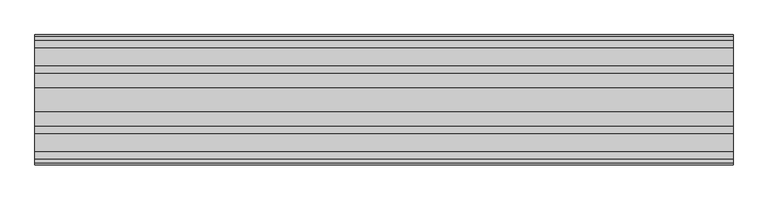
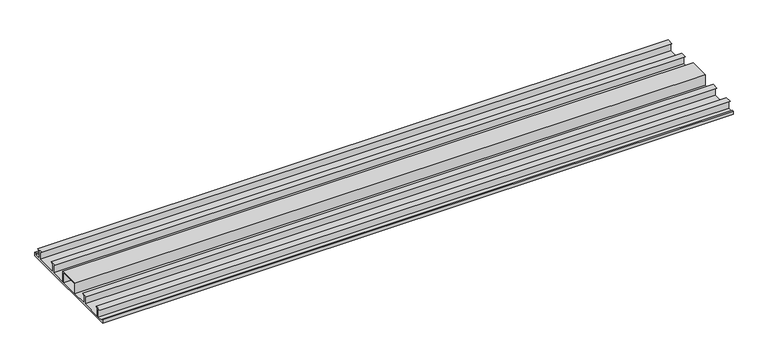
"""IFC4 building model written with IfcOpenShell, lengths in millimetres: proxy geometry, TN_Гидрошпонка ТН Фундамент : Гидрошпонка ТН Фундамент ДШ-Н-280."""

from ifc_helpers import new_model, si_unit, frame, origin, place, context, project, spatial, polyline, outline, extrude, source, transform, mapped, element, save


def specialty_equipment_545e47b4(model_context):
    return source(origin(), model_context, "Body", "SweptSolid", [
        extrude(outline(polyline([(140.0, 0.0), (-140.0, 0.0), (-140.0, 7.9804873), (-137.0, 7.9804873), (-137.0, 4.0), (-122.0456593, 4.0), (-122.0456593, 22.012356), (-127.5, 25.0), (-112.5, 25.0), (-117.9543407, 22.012356), (-117.9543407, 4.0), (-67.0456593, 4.0), (-67.0456593, 22.012356), (-72.5, 25.0), (-57.5, 25.0), (-62.9543407, 22.012356), (-62.9543407, 4.0), (-25.0, 4.0), (-25.0, 30.0), (25.0, 30.0), (25.0, 4.0), (62.9543407, 4.0), (62.9543407, 22.012356), (57.5, 25.0), (72.5, 25.0), (67.0456593, 22.012356), (67.0456593, 4.0), (117.9543407, 4.0), (117.9543407, 22.012356), (112.5, 25.0), (127.5, 25.0), (122.0456593, 22.012356), (122.0456593, 4.0), (137.0, 4.0), (137.0, 7.9804873), (140.0, 7.9804873), (140.0, 0.0)]), holes=[polyline([(-22.0213922, 27.012356), (-22.0213922, 2.7793951), (22.0213922, 2.7793951), (22.0213922, 27.012356), (-22.0213922, 27.012356)])]), frame((0.0, 0.0, 0.0), z_axis=(1.0, 0.0, 0.0), x_axis=(0.0, 1.0, 0.0)), (0.0, 0.0, 1.0), 1500.0),
    ])


if __name__ == "__main__":
    model = new_model("IFC4")
    model_context = context("Model", 3, world=origin())
    ifc_project = project(units=[si_unit("LENGTHUNIT", "METRE", prefix="MILLI")], contexts=[model_context])
    site = spatial("IfcSite", under=ifc_project)
    building = spatial("IfcBuilding", under=site)
    placement = place(None, origin())
    specialty_equipment_shape = specialty_equipment_545e47b4(model_context)
    element("IfcBuildingElementProxy", 1, Name="TN_Гидрошпонка ТН Фундамент : Гидрошпонка ТН Фундамент ДШ-Н-280", ObjectType="TN_Гидрошпонка ТН Фундамент : Гидрошпонка ТН Фундамент ДШ-Н-280", at=placement, inside=building, context=model_context, shape_type="MappedRepresentation", body=[
        mapped(specialty_equipment_shape, transform((0.0, 0.0, 0.0), x_axis=(1.0, 0.0, 0.0), y_axis=(0.0, 1.0, 0.0), z_axis=(0.0, 0.0, 1.0))),
    ])
    save(model, "model.ifc")

# Revit data of these elements
# Type "TN_Гидрошпонка ТН Фундамент : Гидрошпонка ТН Фундамент ДШ-Н-280"
#   Description = "Наружные гидроизоляционные шпонки ТН Фундамент ДШ-Н предназначены для герметизации деформационных швов бетонирования при строительстве подземных и заглубленных конструкций зданий и сооружений различного назначения и класса ответственности."
#   Type Comments = "п.м."
#   Manufacturer = "ТехноНИКОЛЬ"
#   URL = "https://nav.tn.ru/catalog/gidroizolyatsiya/komplektatsiya-dlya-gidroizolyatsii/gidroshponki-tekhnonikol-fundament-dsh-n/"
#   ADSK_Примечание = ""
#   ADSK_Обозначение [instance default] = "ТехноНИКОЛЬ"
#   ADSK_Наименование = "Гидрошпонка ТН Фундамент ДШ-Н-280"
#   ADSK_Масса_Текст = ""
#   ADSK_Марка = ""
#   ADSK_Код изделия = "66672"
#   ADSK_Завод-изготовитель [instance default] = "ТехноНИКОЛЬ"
#   ADSK_Единица измерения [instance default] = "п.м."
#   ADSK_Группирование = "Гидрошпонки"
#   ADSK_URL страницы изделия = "https://nav.tn.ru/catalog/gidroizolyatsiya/komplektatsiya-dlya-gidroizolyatsii/gidroshponki-tekhnonikol-fundament-dsh-n/"
#   ADSK_URL документации изделия = "https://nav.tn.ru/upload/iblock/ec5/xbb24x1u8yp3edzrrex0jfnnntpjibsj/Tekhlist-7.399_Gidroshponki-TN-Fundament-DSH_N_RU_ru.pdf"
#   built-in parameter 1001306 [instance default] = 3.28084 (stored number, unit not read)
#   ADSK_Размер_Длина [instance default] = 1000 mm
#   ADSK_Количество [instance default] = 1
#   Гидрошпонка ТН Фундамент ТШ-Н-210 = no
#   Гидрошпонка ТН Фундамент ДШП-В-50 = no
#   Гидрошпонка ТН Фундамент ДШП-В-20 = no
#   Гидрошпонка ТН Фундамент ДШ-В-280 = no
#   Гидрошпонка ТН Фундамент ДШ-В-250 = no
#   Гидрошпонка ТН Фундамент ТШ-В-250 = no
#   Гидрошпонка ТН Фундамент ТПС-В 140-1 = no
#   Гидрошпонка ТН Фундамент ДШ-Н-280 = yes
#   Гидрошпонка ТН Фундамент ДШ-Н-250 = no
#   Гидрошпонка ТН Фундамент ТПС-В 100-2 = no
#   Гидрошпонка ТН Фундамент ТШ-Н-250 = no
#   Гидрошпонка ТН Фундамент ТШ-В-210 = no
#   Материал = TN_ПВХ_Черный
#   Default Elevation = 0
# Element 1 (IfcBuildingElementProxy, "TN_Гидрошпонка ТН Фундамент : Гидрошпонка ТН Фундамент ДШ-Н-280")
#   built-in parameter 1001306 = 4.92126 (stored number, unit not read)
#   ADSK_Размер_Длина = 1500 mm
#   ADSK_Количество = 1.5
#   Materials on its faces: "TN_ПВХ_Черный"
# Materials
#   "TN_ПВХ_Черный": class "Типовые", colour RGB 48 48 48, transparency 0, Cost = 0
